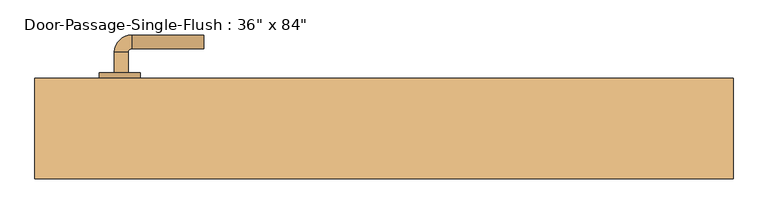
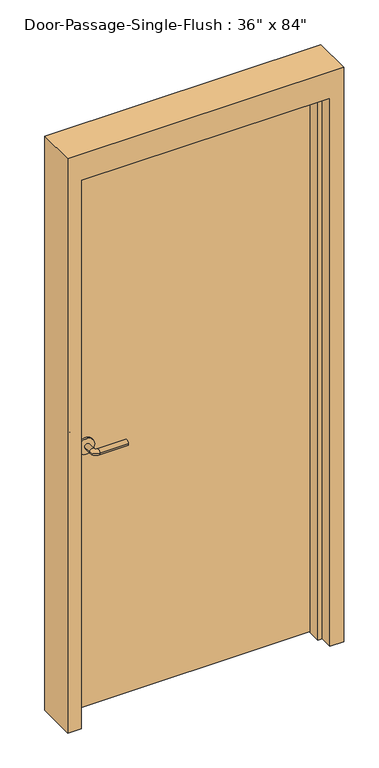
"""IFC4 building model written with IfcOpenShell, lengths in millimetres: door geometry."""

import ifcopenshell
import ifcopenshell.guid

model = None  # the IFC model being written
_history = None  # IfcOwnerHistory: only IFC2X3 demands one
_inside = {}  # id of a spatial element -> (the spatial element, [elements in it])
_under = {}  # id of a project, library or spatial element -> (it, [spatial elements below it])
_declared = {}  # id of a project -> (the project, [libraries it declares])
_typed = {}  # id of a type object -> (the type object, [elements of that type])
_made_of = {}  # id of a material, layer set ... -> (it, [elements and type objects made of it])


def new_model(schema):
    """Start an empty IFC model of exactly this schema.

    Asked for "IFC4X3", IfcOpenShell would pick the latest addendum, in which some entities
    have other attributes; the version numbers below select the first issue.
    IFC2X3 requires an IfcOwnerHistory on every rooted entity: one is made here for all.
    """
    global model, _history
    if schema == "IFC4X3":
        model = ifcopenshell.file(schema_version=(4, 3, 0, 0))
    else:
        model = ifcopenshell.file(schema=schema)
    _inside.clear()
    _under.clear()
    _declared.clear()
    _typed.clear()
    _made_of.clear()
    _history = None
    if model.schema == "IFC2X3":
        org = make("IfcOrganization", Name="unknown")
        user = make(
            "IfcPersonAndOrganization",
            ThePerson=make("IfcPerson", FamilyName="unknown"),
            TheOrganization=org,
        )
        app = make(
            "IfcApplication",
            ApplicationDeveloper=org,
            Version="unknown",
            ApplicationFullName="unknown",
            ApplicationIdentifier="unknown",
        )
        _history = make(
            "IfcOwnerHistory",
            OwningUser=user,
            OwningApplication=app,
            ChangeAction="ADDED",
            CreationDate=0,
        )
    return model


def make(cls, **values):
    """One entity of the class cls with the attributes given. An attribute that is None is left unset."""
    return model.create_entity(
        cls, **{name: value for name, value in values.items() if value is not None}
    )


def rooted(cls, **values):
    """An entity with a GlobalId (a new one), such as an element, a storey or a relation."""
    return make(cls, GlobalId=ifcopenshell.guid.new(), OwnerHistory=_history, **values)


def si_unit(unit_type, name, prefix=None):
    """IfcSIUnit, for example si_unit("LENGTHUNIT", "METRE", prefix="MILLI")."""
    return make("IfcSIUnit", UnitType=unit_type, Prefix=prefix, Name=name)


def assignment(units):
    """IfcUnitAssignment: the units of a project."""
    return None if units is None else make("IfcUnitAssignment", Units=units)


def point(xyz):
    """IfcCartesianPoint."""
    return None if xyz is None else make("IfcCartesianPoint", Coordinates=xyz)


def direction(xyz):
    """IfcDirection."""
    return None if xyz is None else make("IfcDirection", DirectionRatios=xyz)


def frame(location, z_axis=None, x_axis=None):
    """IfcAxis2Placement3D, a coordinate frame: its origin and axes. An axis left out is left unset."""
    return make(
        "IfcAxis2Placement3D",
        Location=point(location),
        Axis=direction(z_axis),
        RefDirection=direction(x_axis),
    )


def frame_2d(location, x_axis=None):
    """IfcAxis2Placement2D, a coordinate frame in the plane: its origin and x axis."""
    return make(
        "IfcAxis2Placement2D", Location=point(location), RefDirection=direction(x_axis)
    )


def origin():
    """The frame at (0, 0, 0) with its axes left unset."""
    return frame((0.0, 0.0, 0.0))


def origin_with_axes():
    """The frame at (0, 0, 0) with the z axis (0, 0, 1) and the x axis (1, 0, 0) written out."""
    return frame((0.0, 0.0, 0.0), z_axis=(0.0, 0.0, 1.0), x_axis=(1.0, 0.0, 0.0))


def place(relative_to, where):
    """IfcLocalPlacement: puts the frame where relative to a parent placement (None: the world)."""
    return make(
        "IfcLocalPlacement", PlacementRelTo=relative_to, RelativePlacement=where
    )


def context(
    kind, dimensions, precision=None, world=None, true_north=None, identifier=None
):
    """IfcGeometricRepresentationContext, for example the 3D "Model" context."""
    return make(
        "IfcGeometricRepresentationContext",
        ContextIdentifier=identifier,
        ContextType=kind,
        CoordinateSpaceDimension=dimensions,
        Precision=precision,
        WorldCoordinateSystem=world,
        TrueNorth=true_north,
    )


def project(units=None, contexts=None):
    """IfcProject with its units and contexts."""
    return rooted(
        "IfcProject",
        Name="project",
        RepresentationContexts=contexts,
        UnitsInContext=assignment(units),
    )


def spatial(cls, under=None, at=None, **own):
    """A site, building, storey or space (cls), placed at a placement, below another one or the project."""
    s = rooted(cls, ObjectPlacement=at, **own)
    if under is not None:
        _under.setdefault(under.id(), (under, []))[1].append(s)
    return s


def polyline(points):
    """IfcPolyline through the points."""
    return make("IfcPolyline", Points=[point(p) for p in points])


def circle_curve(where, radius):
    """IfcCircle in the frame where."""
    return make("IfcCircle", Position=where, Radius=radius)


def ellipse_curve(where, semi_axis1, semi_axis2):
    """IfcEllipse in the frame where."""
    return make(
        "IfcEllipse", Position=where, SemiAxis1=semi_axis1, SemiAxis2=semi_axis2
    )


def trimmed(basis, trim1, trim2, sense, master):
    """IfcTrimmedCurve: the piece of a basis curve between two trims."""
    return make(
        "IfcTrimmedCurve",
        BasisCurve=basis,
        Trim1=trim1,
        Trim2=trim2,
        SenseAgreement=sense,
        MasterRepresentation=master,
    )


def segment(curve, same_sense, transition):
    """IfcCompositeCurveSegment."""
    return make(
        "IfcCompositeCurveSegment",
        Transition=transition,
        SameSense=same_sense,
        ParentCurve=curve,
    )


def composite_curve(segments, self_intersect=None):
    """IfcCompositeCurve: segments joined end to end."""
    return make("IfcCompositeCurve", Segments=segments, SelfIntersect=self_intersect)


def outline(outer, holes=None, kind="AREA"):
    """IfcArbitraryClosedProfileDef: a profile drawn as a closed curve; with holes, ...WithVoids."""
    if holes is None:
        return make("IfcArbitraryClosedProfileDef", ProfileType=kind, OuterCurve=outer)
    return make(
        "IfcArbitraryProfileDefWithVoids",
        ProfileType=kind,
        OuterCurve=outer,
        InnerCurves=holes,
    )


def extrude(swept, where, along, depth):
    """IfcExtrudedAreaSolid: the profile swept, set in the frame where, extruded along a direction by depth."""
    return make(
        "IfcExtrudedAreaSolid",
        SweptArea=swept,
        Position=where,
        ExtrudedDirection=direction(along),
        Depth=depth,
    )


def faces_of(points, faces, orient=None, outer=None):
    """IfcFace entities. A face is a list of loops; a loop is a list of indices into points, from 0.

    orient and outer hold one flag for each loop. By default every Orientation is true, the
    first loop of a face is its IfcFaceOuterBound and the others are IfcFaceBound.
    """
    made = []
    for i, loops in enumerate(faces):
        bounds = []
        for j, loop in enumerate(loops):
            is_outer = j == 0 if outer is None else outer[i][j]
            bounds.append(
                make(
                    "IfcFaceOuterBound" if is_outer else "IfcFaceBound",
                    Bound=make("IfcPolyLoop", Polygon=[points[k] for k in loop]),
                    Orientation=True if orient is None else orient[i][j],
                )
            )
        made.append(make("IfcFace", Bounds=bounds))
    return made


def faceted_brep(points, faces, orient=None, outer=None, voids=None):
    """IfcFacetedBrep: a solid bounded by flat faces; with voids (closed shells), ...WithVoids."""
    shared = [point(p) for p in points]
    hull = make("IfcClosedShell", CfsFaces=faces_of(shared, faces, orient, outer))
    if voids is None:
        return make("IfcFacetedBrep", Outer=hull)
    return make(
        "IfcFacetedBrepWithVoids",
        Outer=hull,
        Voids=[
            make(cls, CfsFaces=faces_of(shared, fs, o, b)) for cls, fs, o, b in voids
        ],
    )


def shape(context_of_items, identifier, shape_type, items):
    """IfcShapeRepresentation: the items that make up one representation, for example the "Body"."""
    return make(
        "IfcShapeRepresentation",
        ContextOfItems=context_of_items,
        RepresentationIdentifier=identifier,
        RepresentationType=shape_type,
        Items=items,
    )


def source(mapping_origin, context_of_items, identifier, shape_type, items):
    """IfcRepresentationMap: a shape defined once, which mapped items show again and again."""
    return make(
        "IfcRepresentationMap",
        MappingOrigin=mapping_origin,
        MappedRepresentation=shape(context_of_items, identifier, shape_type, items),
    )


def transform(
    local_origin,
    x_axis=None,
    y_axis=None,
    z_axis=None,
    scale=None,
    scale2=None,
    scale3=None,
    uniform=True,
):
    """IfcCartesianTransformationOperator3D, or its non-uniform kind. x_axis, y_axis, z_axis: its Axis1, 2, 3."""
    if uniform:
        return make(
            "IfcCartesianTransformationOperator3D",
            Axis1=direction(x_axis),
            Axis2=direction(y_axis),
            LocalOrigin=point(local_origin),
            Scale=scale,
            Axis3=direction(z_axis),
        )
    return make(
        "IfcCartesianTransformationOperator3DnonUniform",
        Axis1=direction(x_axis),
        Axis2=direction(y_axis),
        LocalOrigin=point(local_origin),
        Scale=scale,
        Axis3=direction(z_axis),
        Scale2=scale2,
        Scale3=scale3,
    )


def mapped(mapping_source, mapping_target):
    """IfcMappedItem: shows the shape of a source again, moved by a transform."""
    return make(
        "IfcMappedItem", MappingSource=mapping_source, MappingTarget=mapping_target
    )


def made_of(thing, what):
    """Note that an element or type object is made of a material, layer set ...; save() writes the relation."""
    if what is not None:
        _made_of.setdefault(what.id(), (what, []))[1].append(thing)
    return thing


def element(
    cls,
    number,
    at=None,
    inside=None,
    cuts=None,
    type_object=None,
    material=None,
    context=None,
    identifier="Body",
    shape_type=None,
    held_by="IfcProductDefinitionShape",
    body=None,
    shapes=None,
    **own,
):
    """One element of the class cls, such as IfcWall. Its Tag is "e" and its number.

    at: its placement. inside: the storey or other place that contains it. cuts: it is an
    opening in that element (IfcRelVoidsElement). A single representation is given by context,
    identifier, shape_type and body (its items); several are given by shapes. held_by: the class
    of the entity that holds the representations. save() writes the other relations.
    """
    e = rooted(cls, Tag="e%d" % number, ObjectPlacement=at, **own)
    if body is not None:
        shapes = [shape(context, identifier, shape_type, body)]
    if shapes is not None:
        e.Representation = make(held_by, Representations=shapes)
    if inside is not None:
        _inside.setdefault(inside.id(), (inside, []))[1].append(e)
    if cuts is not None:
        rooted(
            "IfcRelVoidsElement", RelatingBuildingElement=cuts, RelatedOpeningElement=e
        )
    if type_object is not None:
        _typed.setdefault(type_object.id(), (type_object, []))[1].append(e)
    return made_of(e, material)


def aggregate(whole, parts):
    """IfcRelAggregates: a whole, such as a stair, and the parts it consists of."""
    return rooted("IfcRelAggregates", RelatingObject=whole, RelatedObjects=parts)


def save(model, path):
    """Write the relations noted so far, then the file.

    IfcRelAggregates (storeys below a building ...), IfcRelContainedInSpatialStructure (elements
    in a storey), IfcRelDefinesByType, IfcRelAssociatesMaterial and IfcRelDeclares: one each for
    every whole, place, type object, material and project.
    """
    for whole, parts in _under.values():
        aggregate(whole, parts)
    for where, things in _inside.values():
        rooted(
            "IfcRelContainedInSpatialStructure",
            RelatedElements=things,
            RelatingStructure=where,
        )
    for kind, things in _typed.values():
        rooted("IfcRelDefinesByType", RelatedObjects=things, RelatingType=kind)
    for what, things in _made_of.values():
        rooted("IfcRelAssociatesMaterial", RelatedObjects=things, RelatingMaterial=what)
    for by, libraries in _declared.values():
        rooted("IfcRelDeclares", RelatingContext=by, RelatedDefinitions=libraries)
    model.write(path)


def plane_surface(at):
    """IfcPlane: the flat surface through the origin of the frame at, square to its z axis."""
    return make("IfcPlane", Position=at)


def cylinder_surface(at, radius):
    """IfcCylindricalSurface: all points at the distance radius from the z axis of the frame at."""
    return make("IfcCylindricalSurface", Position=at, Radius=radius)


def revolved_surface(curve, axis_point, axis_direction):
    """IfcSurfaceOfRevolution: the curve turned about the line through axis_point along axis_direction."""
    return make(
        "IfcSurfaceOfRevolution",
        SweptCurve=make("IfcArbitraryOpenProfileDef", ProfileType="CURVE", Curve=curve),
        AxisPosition=make("IfcAxis1Placement", Location=point(axis_point), Axis=direction(axis_direction)),
    )


def advanced_brep(points, edges, surfaces, faces):
    """IfcAdvancedBrep: a solid bounded by faces that lie on surfaces and meet in shared edges.

    An edge is (start, end): straight between two places in points (the first is 0);
    or (start, end, curve); or (start, end, curve, False) where it runs against its curve.
    A face is (place in surfaces, loops), or (place, loops, False) where it looks against
    its surface's normal. A loop lists edges by number (the first is 1), with a minus sign
    where the edge is run from its end to its start. The first loop is the outer one.
    """
    corners = [point(p) for p in points]
    vertices = [make("IfcVertexPoint", VertexGeometry=c) for c in corners]
    made = []
    for start, end, *more in edges:
        made.append(
            make(
                "IfcEdgeCurve",
                EdgeStart=vertices[start],
                EdgeEnd=vertices[end],
                EdgeGeometry=more[0] if more else make("IfcPolyline", Points=[corners[start], corners[end]]),
                SameSense=more[1] if len(more) > 1 else True,
            )
        )
    hull = []
    for where, loops, *sense in faces:
        bounds = []
        for j, loop in enumerate(loops):
            ring = [make("IfcOrientedEdge", EdgeElement=made[abs(k) - 1], Orientation=k > 0) for k in loop]
            bounds.append(
                make(
                    "IfcFaceOuterBound" if j == 0 else "IfcFaceBound",
                    Bound=make("IfcEdgeLoop", EdgeList=ring),
                    Orientation=True,
                )
            )
        hull.append(make("IfcAdvancedFace", Bounds=bounds, FaceSurface=surfaces[where], SameSense=sense[0] if sense else True))
    return make("IfcAdvancedBrep", Outer=make("IfcClosedShell", CfsFaces=hull))


def door_a856c21e(model_context):
    return source(origin(), model_context, "Body", "SolidModel", [
        advanced_brep(
        [(-392.190625, 80.9, 1016.0), (-372.190625, 80.9, 1016.0), (-372.190625, 50.9, 1016.0), (-392.190625, 50.9, 1016.0), (-367.190625, 45.9, 1016.0), (-367.190625, 25.9, 1016.0), (-262.190625, 25.9, 1016.0), (-262.190625, 45.9, 1016.0)],
        [
            (0, 1, circle_curve(frame((-382.190625, 80.9, 1016.0), z_axis=(0.0, 1.0, 0.0), x_axis=(1.0, 0.0, 0.0)), 10.0)),
            (1, 0, circle_curve(frame((-382.190625, 80.9, 1016.0), z_axis=(0.0, 1.0, 0.0), x_axis=(1.0, 0.0, 0.0)), 10.0)),
            (1, 2),
            (2, 3, circle_curve(frame((-382.190625, 50.9, 1016.0), z_axis=(0.0, 1.0, 0.0), x_axis=(1.0, 0.0, 0.0)), 10.0)),
            (3, 0),
            (3, 2, circle_curve(frame((-382.190625, 50.9, 1016.0), z_axis=(0.0, 1.0, 0.0), x_axis=(1.0, 0.0, 0.0)), 10.0)),
            (4, 5, circle_curve(frame((-367.190625, 35.9, 1016.0), z_axis=(-1.0, 0.0, 0.0), x_axis=(0.0, 1.0, 0.0)), 10.0)),
            (5, 3, circle_curve(frame((-367.190625, 50.9, 1016.0), z_axis=(0.0, 0.0, -1.0), x_axis=(-1.0, 0.0, 0.0)), 25.0)),
            (2, 4, circle_curve(frame((-367.190625, 50.9, 1016.0), z_axis=(0.0, 0.0, 1.0), x_axis=(-1.0, 0.0, 0.0)), 5.0)),
            (5, 4, circle_curve(frame((-367.190625, 35.9, 1016.0), z_axis=(-1.0, 0.0, 0.0), x_axis=(0.0, 1.0, 0.0)), 10.0)),
            (6, 7, circle_curve(frame((-262.190625, 35.9, 1016.0), z_axis=(1.0, 0.0, 0.0), x_axis=(0.0, 1.0, 0.0)), 10.0)),
            (7, 6, circle_curve(frame((-262.190625, 35.9, 1016.0), z_axis=(1.0, 0.0, 0.0), x_axis=(0.0, 1.0, 0.0)), 10.0)),
            (4, 7),
            (6, 5),
        ],
        [
            plane_surface(frame((-382.190625, 80.9, 1016.0), z_axis=(0.0, 1.0, 0.0), x_axis=(0.0, 0.0, 1.0))),
            cylinder_surface(frame((-382.190625, 80.9, 1016.0), z_axis=(0.0, 1.0, 0.0), x_axis=(1.0, 0.0, 0.0)), 10.0),
            revolved_surface(trimmed(ellipse_curve(frame((-382.190625, 50.9, 1016.0), z_axis=(0.0, -1.0, 0.0), x_axis=(1.0, 0.0, 0.0)), 10.0, 10.0), [point((-392.190625, 50.9, 1016.0))], [point((-372.190625, 50.9, 1016.0))], True, "CARTESIAN"), (-367.190625, 50.9, 1016.0), (0.0, 0.0, -1.0)),
            revolved_surface(trimmed(ellipse_curve(frame((-382.190625, 50.9, 1016.0), z_axis=(0.0, -1.0, 0.0), x_axis=(1.0, 0.0, 0.0)), 10.0, 10.0), [point((-372.190625, 50.9, 1016.0))], [point((-392.190625, 50.9, 1016.0))], True, "CARTESIAN"), (-367.190625, 50.9, 1016.0), (0.0, 0.0, -1.0)),
            plane_surface(frame((-262.190625, 35.9, 1016.0), z_axis=(1.0, 0.0, 0.0), x_axis=(0.0, 0.0, 1.0))),
            cylinder_surface(frame((-367.190625, 35.9, 1016.0), z_axis=(-1.0, 0.0, 0.0), x_axis=(0.0, 1.0, 0.0)), 10.0),
        ],
        [
            (0, [[1, 2]]),
            (1, [[3, 4, 5, -2]]),
            (1, [[-5, 6, -3, -1]]),
            (2, [[7, 8, -4, 9]]),
            (3, [[10, -9, -6, -8]]),
            (4, [[11, 12]]),
            (5, [[13, -11, 14, -7]]),
            (5, [[-14, -12, -13, -10]]),
        ],
    ),
        extrude(outline(composite_curve([segment(trimmed(circle_curve(frame_2d((1016.0, -384.690625)), 30.0), [point((1016.0, -414.690625))], [point((1016.0, -354.690625))], False, "CARTESIAN"), True, "CONTINUOUS"), segment(trimmed(circle_curve(frame_2d((1016.0, -384.690625)), 30.0), [point((1016.0, -354.690625))], [point((1016.0, -414.690625))], False, "CARTESIAN"), True, "CONTINUOUS")], self_intersect=False)), frame((0.0, 80.9, 0.0), z_axis=(0.0, 1.0, 0.0), x_axis=(0.0, 0.0, 1.0)), (0.0, 0.0, 1.0), 8.0),
        advanced_brep(
        [(-392.190625, 141.35, 1016.0), (-372.190625, 141.35, 1016.0), (-392.190625, 171.35, 1016.0), (-372.190625, 171.35, 1016.0), (-367.190625, 176.35, 1016.0), (-367.190625, 196.35, 1016.0), (-262.190625, 196.35, 1016.0), (-262.190625, 176.35, 1016.0)],
        [
            (0, 1, circle_curve(frame((-382.190625, 141.35, 1016.0), z_axis=(0.0, -1.0, 0.0), x_axis=(1.0, 0.0, 0.0)), 10.0)),
            (1, 0, circle_curve(frame((-382.190625, 141.35, 1016.0), z_axis=(0.0, -1.0, 0.0), x_axis=(1.0, 0.0, 0.0)), 10.0)),
            (0, 2),
            (2, 3, circle_curve(frame((-382.190625, 171.35, 1016.0), z_axis=(0.0, -1.0, 0.0), x_axis=(1.0, 0.0, 0.0)), 10.0)),
            (3, 1),
            (3, 2, circle_curve(frame((-382.190625, 171.35, 1016.0), z_axis=(0.0, -1.0, 0.0), x_axis=(1.0, 0.0, 0.0)), 10.0)),
            (4, 3, circle_curve(frame((-367.190625, 171.35, 1016.0), z_axis=(0.0, 0.0, 1.0), x_axis=(-1.0, 0.0, 0.0)), 5.0)),
            (2, 5, circle_curve(frame((-367.190625, 171.35, 1016.0), z_axis=(0.0, 0.0, -1.0), x_axis=(-1.0, 0.0, 0.0)), 25.0)),
            (5, 4, circle_curve(frame((-367.190625, 186.35, 1016.0), z_axis=(-1.0, 0.0, 0.0), x_axis=(0.0, -1.0, 0.0)), 10.0)),
            (4, 5, circle_curve(frame((-367.190625, 186.35, 1016.0), z_axis=(-1.0, 0.0, 0.0), x_axis=(0.0, -1.0, 0.0)), 10.0)),
            (6, 7, circle_curve(frame((-262.190625, 186.35, 1016.0), z_axis=(1.0, 0.0, 0.0), x_axis=(0.0, -1.0, 0.0)), 10.0)),
            (7, 6, circle_curve(frame((-262.190625, 186.35, 1016.0), z_axis=(1.0, 0.0, 0.0), x_axis=(0.0, -1.0, 0.0)), 10.0)),
            (5, 6),
            (7, 4),
        ],
        [
            plane_surface(frame((-382.190625, 141.35, 1016.0), z_axis=(0.0, -1.0, 0.0), x_axis=(0.0, 0.0, 1.0))),
            cylinder_surface(frame((-382.190625, 141.35, 1016.0), z_axis=(0.0, -1.0, 0.0), x_axis=(1.0, 0.0, 0.0)), 10.0),
            revolved_surface(trimmed(ellipse_curve(frame((-382.190625, 171.35, 1016.0), z_axis=(0.0, -1.0, 0.0), x_axis=(1.0, 0.0, 0.0)), 10.0, 10.0), [point((-392.190625, 171.35, 1016.0))], [point((-372.190625, 171.35, 1016.0))], True, "CARTESIAN"), (-367.190625, 171.35, 1016.0), (0.0, 0.0, -1.0)),
            revolved_surface(trimmed(ellipse_curve(frame((-382.190625, 171.35, 1016.0), z_axis=(0.0, -1.0, 0.0), x_axis=(1.0, 0.0, 0.0)), 10.0, 10.0), [point((-372.190625, 171.35, 1016.0))], [point((-392.190625, 171.35, 1016.0))], True, "CARTESIAN"), (-367.190625, 171.35, 1016.0), (0.0, 0.0, -1.0)),
            plane_surface(frame((-262.190625, 186.35, 1016.0), z_axis=(1.0, 0.0, 0.0), x_axis=(0.0, 0.0, 1.0))),
            cylinder_surface(frame((-367.190625, 186.35, 1016.0), z_axis=(-1.0, 0.0, 0.0), x_axis=(0.0, -1.0, 0.0)), 10.0),
        ],
        [
            (0, [[1, 2]]),
            (1, [[-1, 3, 4, 5]]),
            (1, [[-2, -5, 6, -3]]),
            (2, [[7, -4, 8, 9]]),
            (3, [[-8, -6, -7, 10]]),
            (4, [[11, 12]]),
            (5, [[-9, 13, -12, 14]]),
            (5, [[-10, -14, -11, -13]]),
        ],
    ),
        extrude(outline(composite_curve([segment(trimmed(circle_curve(frame_2d((1016.0, -384.690625)), 30.0), [point((1016.0, -414.690625))], [point((1016.0, -354.690625))], False, "CARTESIAN"), True, "CONTINUOUS"), segment(trimmed(circle_curve(frame_2d((1016.0, -384.690625)), 30.0), [point((1016.0, -354.690625))], [point((1016.0, -414.690625))], False, "CARTESIAN"), True, "CONTINUOUS")], self_intersect=False)), frame((0.0, 133.35, 0.0), z_axis=(0.0, 1.0, 0.0), x_axis=(0.0, 0.0, 1.0)), (0.0, 0.0, 1.0), 8.0),
        faceted_brep([(457.2, 84.1375, 0.0), (457.2, 133.35, 0.0), (508.0, 133.35, 0.0), (508.0, -12.7, 0.0), (457.2, -12.7, 0.0), (457.2, 36.5125, 0.0), (441.325, 36.5125, 0.0), (441.325, 84.1375, 0.0), (457.2, 84.1375, 2133.6), (457.2, 133.35, 2133.6), (-457.2, 133.35, 2133.6), (-457.2, 133.35, 0.0), (-508.0, 133.35, 0.0), (-508.0, 133.35, 2235.2), (508.0, 133.35, 2235.2), (508.0, -12.7, 2235.2), (-508.0, -12.7, 2235.2), (-508.0, -12.7, 0.0), (-457.2, -12.7, 0.0), (-457.2, -12.7, 2133.6), (457.2, -12.7, 2133.6), (457.2, 36.5125, 2133.6), (-457.2, 36.5125, 2133.6), (-457.2, 36.5125, 0.0), (-441.325, 36.5125, 0.0), (-441.325, 36.5125, 2117.725), (441.325, 36.5125, 2117.725), (441.325, 84.1375, 2117.725), (-441.325, 84.1375, 2117.725), (-441.325, 84.1375, 0.0), (-457.2, 84.1375, 0.0), (-457.2, 84.1375, 2133.6)], [[[0, 1, 2, 3, 4, 5, 6, 7]], [[1, 0, 8, 9]], [[2, 1, 9, 10, 11, 12, 13, 14]], [[3, 2, 14, 15]], [[4, 3, 15, 16, 17, 18, 19, 20]], [[5, 4, 20, 21]], [[6, 5, 21, 22, 23, 24, 25, 26]], [[7, 6, 26, 27]], [[0, 7, 27, 28, 29, 30, 31, 8]], [[9, 8, 31, 10]], [[20, 19, 22, 21]], [[26, 25, 28, 27]], [[12, 11, 30, 29, 24, 23, 18, 17]], [[11, 10, 31, 30]], [[13, 12, 17, 16]], [[19, 18, 23, 22]], [[25, 24, 29, 28]], [[15, 14, 13, 16]]]),
        extrude(outline(polyline([(457.2, 88.9), (-457.2, 88.9), (-457.2, 133.35), (457.2, 133.35), (457.2, 88.9)])), origin_with_axes(), (0.0, 0.0, 1.0), 2133.6),
    ])


if __name__ == "__main__":
    model = new_model("IFC4")
    model_context = context("Model", 3, world=origin())
    ifc_project = project(units=[si_unit("LENGTHUNIT", "METRE", prefix="MILLI")], contexts=[model_context])
    site = spatial("IfcSite", under=ifc_project)
    building = spatial("IfcBuilding", under=site)
    placement = place(None, origin())
    door_shape = door_a856c21e(model_context)
    element("IfcDoor", 1, ObjectType="Door-Passage-Single-Flush : 36\" x 84\"", at=placement, inside=building, context=model_context, shape_type="MappedRepresentation", body=[
        mapped(door_shape, transform((0.0, 0.0, 0.0), x_axis=(1.0, 0.0, 0.0), y_axis=(0.0, 1.0, 0.0), z_axis=(0.0, 0.0, 1.0))),
    ])
    save(model, "model.ifc")

# Revit data of these elements
# Type "Door-Passage-Single-Flush : 36\" x 84\""
#   Type Mark = "19"
#   Fire Rating = "--"
#   Assembly Code = "B2030200"
#   Analytic Construction = "Wooden"
#   Thickness = 0' - 1 3/4"
#   Thermal Resistance (R) = 2.5876 (h·ft²·°F)/BTU
#   Swing Angle [instance default] = 90.00°
#   Strike Height = 3' - 4"
#   Rough Width [instance default] = 3' - 4"
#   Rough Height [instance default] = 7' - 4"
#   MF Opening Height [instance default] = 0' - 4"
#   MF Opening Width [instance default] = 0' - 4"
#   Inset Calculate [instance default] = 0' - 4"
#   Masonry Inset [instance default] = 0' - 1"
#   Height = 7' - 0"
#   Width = 3' - 0"
#   Heat Transfer Coefficient (U) = 0.3865 BTU/(h·ft²·°F)
#   Masonry Frame Depth = 0' - 5 3/4"
#   Masonry Frame [instance default] = yes
#   Function = 1
#   Dry Wall Frame [instance default] = no
#   Panel Material = Wood - Birch
#   Frame Material = Metal - Paint Finish - Grey
#   Door Handle Material = Aluminum
#   Visual Light Transmittance = 0
#   Solar Heat Gain Coefficient = 0
#   Wall Closure = (empty or 0)
# Element 1 (IfcDoor, "Door-Passage-Single-Flush : 36\" x 84\"")
#   Materials on its faces: "Aluminum", "Metal - Paint Finish - Grey", "Wood - Birch"
# Materials
#   "Wood - Birch": class "Wood", colour RGB 166 116 52, transparency 0, Cost = 0
#   "Metal - Paint Finish - Grey": class "Paint", colour RGB 104 104 104, transparency 0, Cost = 0
#   "Aluminum": class "Metal", colour RGB 247 247 247, transparency 0, Description = "Aluminum 6061", Cost = 0
